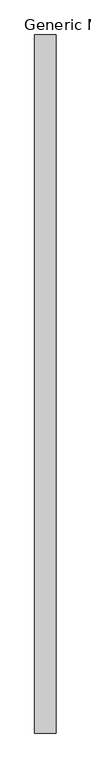
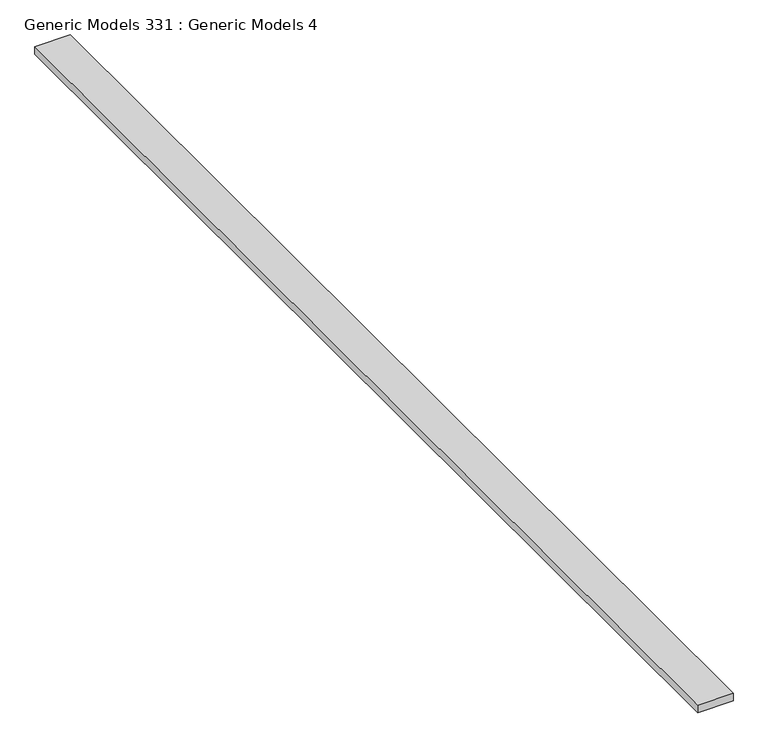
"""IFC4 building model written with IfcOpenShell, lengths in millimetres: proxy geometry, Generic Models 331 : Generic Models 4."""

from ifc_helpers import new_model, si_unit, frame, origin, place, context, project, spatial, polyline, outline, extrude, source, transform, mapped, element, save


def generic_models_331_generic_models_4_795f96d0(model_context):
    return source(origin(), model_context, "Body", "SweptSolid", [
        extrude(outline(polyline([(8553.2763705, -6864.9230338), (8413.5763705, -6864.9230338), (8413.5763704, -2343.7230338), (8553.2763704, -2343.7230338), (8553.2763705, -6864.9230338)])), frame((0.0, 0.0, 126383.796), z_axis=(0.0, 0.0, 1.0), x_axis=(1.0, 0.0, 0.0)), (0.0, 0.0, 1.0), 31.75),
    ])


if __name__ == "__main__":
    model = new_model("IFC4")
    model_context = context("Model", 3, world=origin())
    ifc_project = project(units=[si_unit("LENGTHUNIT", "METRE", prefix="MILLI")], contexts=[model_context])
    site = spatial("IfcSite", under=ifc_project)
    building = spatial("IfcBuilding", under=site)
    placement = place(None, origin())
    generic_models_331_generic_models_4_shape = generic_models_331_generic_models_4_795f96d0(model_context)
    element("IfcBuildingElementProxy", 1, Name="Generic Models 331 : Generic Models 4", ObjectType="Generic Models 331 : Generic Models 4", at=placement, inside=building, context=model_context, shape_type="MappedRepresentation", body=[
        mapped(generic_models_331_generic_models_4_shape, transform((0.0, 0.0, 0.0), x_axis=(1.0, 0.0, 0.0), y_axis=(0.0, 1.0, 0.0), z_axis=(0.0, 0.0, 1.0))),
    ])
    save(model, "model.ifc")

# Revit data of these elements
# Element 1 (IfcBuildingElementProxy, "Generic Models 331 : Generic Models 4")
#   Materials on its faces: "_2X BLOCKING AS REQUIRED"
# Materials
#   "_2X BLOCKING AS REQUIRED": class "Generic", colour RGB 177 130 114, transparency 0, Cost = 0
